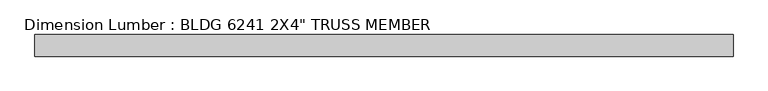
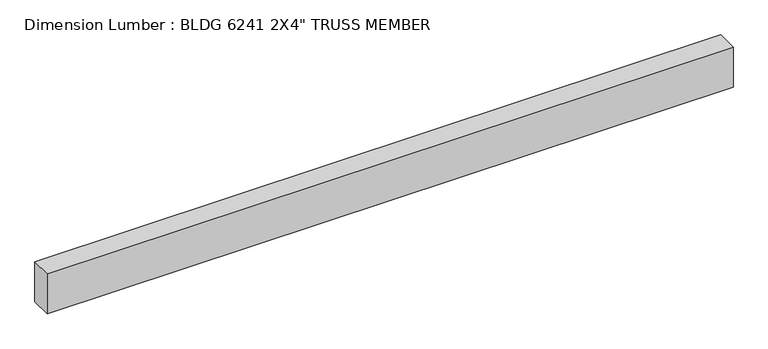
"""IFC4 building model written with IfcOpenShell, lengths in millimetres: beam geometry."""

from ifc_helpers import new_model, si_unit, frame, origin, place, context, project, spatial, polyline, outline, extrude, source, transform, mapped, element, save


def beam_90eea034(model_context):
    return source(origin(), model_context, "Body", "SweptSolid", [
        extrude(outline(polyline([(821.193698, 25.4), (821.193698, -25.4), (-819.5010489, -25.4), (-819.5010489, 25.4), (821.193698, 25.4)])), frame((0.0, 0.0, -50.8), z_axis=(0.0, 0.0, 1.0), x_axis=(1.0, 0.0, 0.0)), (0.0, 0.0, 1.0), 101.6),
    ])


if __name__ == "__main__":
    model = new_model("IFC4")
    model_context = context("Model", 3, world=origin())
    ifc_project = project(units=[si_unit("LENGTHUNIT", "METRE", prefix="MILLI")], contexts=[model_context])
    site = spatial("IfcSite", under=ifc_project)
    building = spatial("IfcBuilding", under=site)
    placement = place(None, origin())
    beam_shape = beam_90eea034(model_context)
    element("IfcBeam", 1, ObjectType="Dimension Lumber : BLDG 6241 2X4\" TRUSS MEMBER", at=placement, inside=building, context=model_context, shape_type="MappedRepresentation", body=[
        mapped(beam_shape, transform((0.0, 0.0, 0.0), x_axis=(1.0, 0.0, 0.0), y_axis=(0.0, 1.0, 0.0), z_axis=(0.0, 0.0, 1.0))),
    ])
    save(model, "model.ifc")

# Revit data of these elements
# Type "Dimension Lumber : BLDG 6241 2X4\" TRUSS MEMBER"
#   Assembly Code = "B10"
#   A = 0.273472 SF
#   Length [instance default] = 5' - 0"
#   b = 0' - 2"
#   d = 0' - 4"
#   Structural Material [instance default] = Softwood, Lumber
# Element 1 (IfcBeam, "Dimension Lumber : BLDG 6241 2X4\" TRUSS MEMBER")
#   Materials on its faces: "Softwood, Lumber"
# Materials
#   "Softwood, Lumber": class "Wood", colour RGB 223 192 134, transparency 0, Description = "Pinus Echinata", Cost = 0
